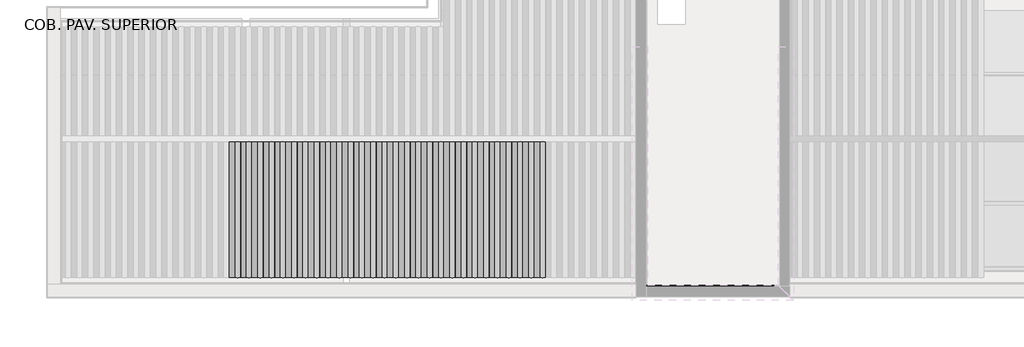
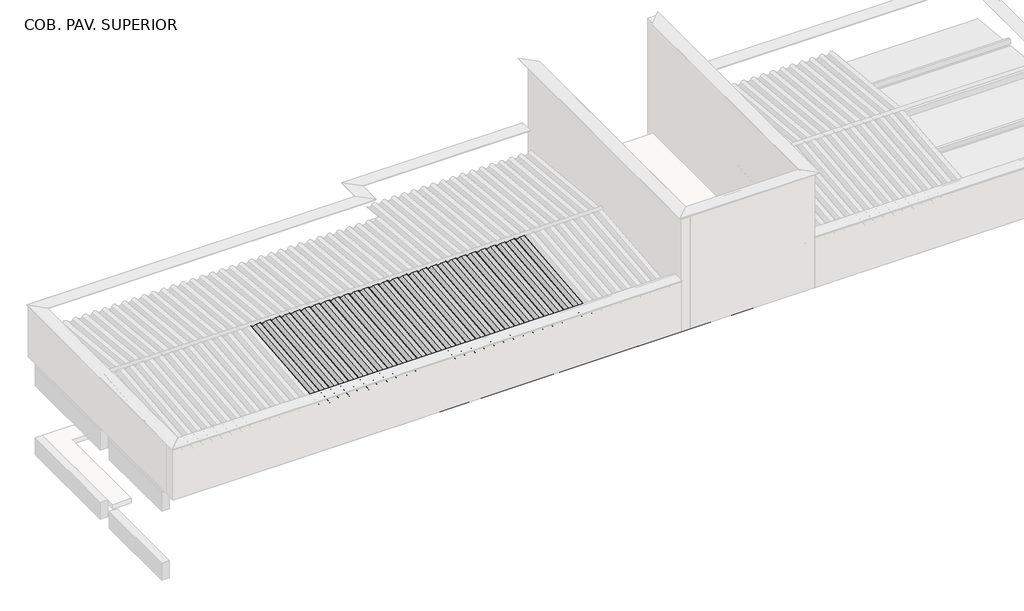
# One storey, part 2 of 7: 38 beams, 9 columns.
# Revit data of these elements (continued)
# Type "Telha Ondulada : Fibrocimento" (continued)
#   Length [instance default] = 1.524 m
#   b = 0.07 m
#   h = 0.16 m
#   Structural Material = .TELHA DE FIBROCIMENTO
#   Assembly Code = ""
# Type "Madeira de lei-Coluna : Pontalete 6X16cm"
#   A = 0.01952 m²
#   b = 0.06 m
#   d = 0.16 m
#   Structural Material [instance default] = none
#   Assembly Code = ""
# Type "TQS - Pilar retangular : 19.0 x 19.0"
#   b = 0.19 m
#   h = 0.19 m
#   Structural Material [instance default] = Concrete - Cast-in-Place Concrete
# Elements 1, 2, 3, 4, 5, 6, 7, 8, 9 (IfcBeam, "Madeira de lei : Berço 6x12cm")
#   Comments = ""
#   Structural Material = .MADEIRAMENTO
#   Phase Created = CC_PE
#   Materials on its faces: ".MADEIRAMENTO"
# Element 10 (IfcBeam, "TQS - Viga retangular : 19.0 x 80.0")
#   Uso = "ESTRUTURA"
#   Titulo = "V410"
#   Chave = "-393"
#   Tipo Elemento = "Viga"
#   SHA1 = "9EB57216FEEAD5BD5BBD6DC7E417A223AA551327"
#   Revisão = ""
#   Tipo de carga = ""
#   Divisor de flexao = ""
#   Secao = ""
#   Configuracao = ""
#   Angulo (graus) = ""
#   Detalhamento = ""
#   Casos de vento manual = ""
#   Tipo = ""
#   Alcas = ""
#   Furos = ""
#   Pino = ""
#   Distribuicao = ""
#   Solidarizado = ""
#   Solidarizar na montagem = ""
#   Unir com o próximo = ""
#   Grupo pre moldado = ""
#   Verificado = ""
#   Concreto C = ""
#   Taxa de armadura (kgf/m³) = 0
#   Carga (tf/m²) = 0
#   Carga (tf/m) = 0
#   Carga (tf) = 0
#   Altura = 0.80 m
#   Rebaixo = -0.60 m
#   Largura = 0.19 m
#   Distancia a face = 0.00 m
#   Distancia ao eixo = 0.00 m
#   Altura gerber esquerda = 0.00 m
#   Largura gerber esquerda = 0.00 m
#   Altura gerber direita = 0.00 m
#   Largura gerber direita = 0.00 m
#   Resultado de Ensaios fck (MPa) = 0
#   Unique TQS ID = -393
#   Principal = yes
#   Structural Material = none
#   Phase Created = CC_PE
# Elements 11, 12, 13, 14, 15, 16, 17, 18, 19, 20, 21, 22, 23, 24, 25, 26, 27, 28, 29, 30, 31, 32, 33, 34, 35, 36, 37, 38 (IfcBeam, "Telha Ondulada : Fibrocimento")
#   Phase Created = CC_PE
#   Materials on its faces: ".TELHA DE FIBROCIMENTO"
# Elements 39, 40, 41, 42, 43, 44, 45, 46 (IfcColumn, "Madeira de lei-Coluna : Pontalete 6X16cm")
#   Comments = ""
#   Structural Material = .MADEIRAMENTO
#   Phase Created = CC_PE
#   Materials on its faces: ".MADEIRAMENTO"
# Element 47 (IfcColumn, "TQS - Pilar retangular : 19.0 x 19.0")
#   Uso = "ESTRUTURA"
#   Titulo = "PT2"
#   Chave = "PT2//0"
#   Tipo Elemento = "Pilar"
#   SHA1 = "F43D605D1DA00D757641A848CE7023BEF37C9FDC"
#   Revisão = ""
#   Tipo de carga = ""
#   Divisor de flexao = ""
#   Secao = "R 19/30 90°"
#   Configuracao = ""
#   Angulo (graus) = ""
#   Detalhamento = ""
#   Casos de vento manual = ""
#   Tipo = ""
#   Alcas = ""
#   Furos = ""
#   Pino = ""
#   Distribuicao = ""
#   Solidarizado = ""
#   Solidarizar na montagem = ""
#   Unir com o próximo = ""
#   Grupo pre moldado = ""
#   Verificado = ""
#   Concreto C = ""
#   Taxa de armadura (kgf/m³) = 0
#   Carga (tf/m²) = 0
#   Carga (tf/m) = 0
#   Carga (tf) = 0
#   Altura = 2.10 m
#   Rebaixo = 0.00 m
#   Altura da fundacao = 0.00 m
#   Largura = 0.00 m
#   Distancia a face = 0.00 m
#   Distancia ao eixo = 0.00 m
#   Resultado de Ensaios fck (MPa) = 0
#   Unique TQS ID = -428
#   Principal = yes
#   Nasce = yes
#   Morre = yes
#   Cabeca de Pilar = no
#   Structural Material = Concrete - Cast-in-Place Concrete
#   Phase Created = CC_PE
#   Materials on its faces: "Concrete - Cast-in-Place Concrete"
# Materials
#   ".TELHA DE FIBROCIMENTO": class "CC_TELHADO", colour RGB 77 77 76, transparency 0, Description = "TELHA ONDULADA FIBROCIMENTO", Cost = 0
#   "Concrete - Cast-in-Place Concrete": class "Unassigned", colour RGB 192 192 192, transparency 0
#   ".MADEIRAMENTO": class ".CC_MADEIRAS", colour RGB 212 179 113, transparency 0, Cost = 0
